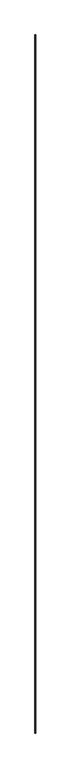
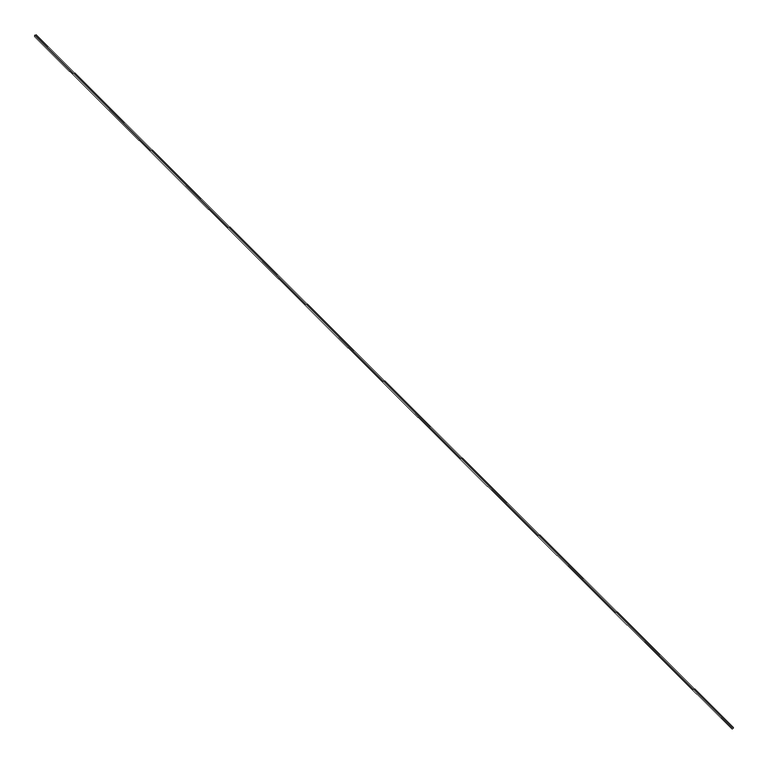
"""IFC4 building model written with IfcOpenShell, lengths in millimetres: proxy geometry, Inner panel:Inner panel:1:Inner panel:1 : Inner panel:Inner panel:300324:2:Inner panel:1:Inner panel:1 : Inner panel:Inner panel:300324:2 : Inner panel:Inner panel:1:Inner panel:1 : Inner panel:Inner panel:300324:300043:57 : Inner panel:Inner panel:1:Inner panel:1 : Inner panel:Inner panel:300324:2:Inner panel:1:Inner panel:1 : Inner panel:Inner panel:300324:2 : Inner panel:Inner panel:1:Inner panel:1 : Inner panel:Inner panel:300324:300043:308120."""

import ifcopenshell
import ifcopenshell.guid

model = None  # the IFC model being written
_history = None  # IfcOwnerHistory: only IFC2X3 demands one
_inside = {}  # id of a spatial element -> (the spatial element, [elements in it])
_under = {}  # id of a project, library or spatial element -> (it, [spatial elements below it])
_declared = {}  # id of a project -> (the project, [libraries it declares])
_typed = {}  # id of a type object -> (the type object, [elements of that type])
_made_of = {}  # id of a material, layer set ... -> (it, [elements and type objects made of it])


def new_model(schema):
    """Start an empty IFC model of exactly this schema.

    Asked for "IFC4X3", IfcOpenShell would pick the latest addendum, in which some entities
    have other attributes; the version numbers below select the first issue.
    IFC2X3 requires an IfcOwnerHistory on every rooted entity: one is made here for all.
    """
    global model, _history
    if schema == "IFC4X3":
        model = ifcopenshell.file(schema_version=(4, 3, 0, 0))
    else:
        model = ifcopenshell.file(schema=schema)
    _inside.clear()
    _under.clear()
    _declared.clear()
    _typed.clear()
    _made_of.clear()
    _history = None
    if model.schema == "IFC2X3":
        org = make("IfcOrganization", Name="unknown")
        user = make(
            "IfcPersonAndOrganization",
            ThePerson=make("IfcPerson", FamilyName="unknown"),
            TheOrganization=org,
        )
        app = make(
            "IfcApplication",
            ApplicationDeveloper=org,
            Version="unknown",
            ApplicationFullName="unknown",
            ApplicationIdentifier="unknown",
        )
        _history = make(
            "IfcOwnerHistory",
            OwningUser=user,
            OwningApplication=app,
            ChangeAction="ADDED",
            CreationDate=0,
        )
    return model


def make(cls, **values):
    """One entity of the class cls with the attributes given. An attribute that is None is left unset."""
    return model.create_entity(
        cls, **{name: value for name, value in values.items() if value is not None}
    )


def rooted(cls, **values):
    """An entity with a GlobalId (a new one), such as an element, a storey or a relation."""
    return make(cls, GlobalId=ifcopenshell.guid.new(), OwnerHistory=_history, **values)


def si_unit(unit_type, name, prefix=None):
    """IfcSIUnit, for example si_unit("LENGTHUNIT", "METRE", prefix="MILLI")."""
    return make("IfcSIUnit", UnitType=unit_type, Prefix=prefix, Name=name)


def assignment(units):
    """IfcUnitAssignment: the units of a project."""
    return None if units is None else make("IfcUnitAssignment", Units=units)


def point(xyz):
    """IfcCartesianPoint."""
    return None if xyz is None else make("IfcCartesianPoint", Coordinates=xyz)


def direction(xyz):
    """IfcDirection."""
    return None if xyz is None else make("IfcDirection", DirectionRatios=xyz)


def frame(location, z_axis=None, x_axis=None):
    """IfcAxis2Placement3D, a coordinate frame: its origin and axes. An axis left out is left unset."""
    return make(
        "IfcAxis2Placement3D",
        Location=point(location),
        Axis=direction(z_axis),
        RefDirection=direction(x_axis),
    )


def origin():
    """The frame at (0, 0, 0) with its axes left unset."""
    return frame((0.0, 0.0, 0.0))


def place(relative_to, where):
    """IfcLocalPlacement: puts the frame where relative to a parent placement (None: the world)."""
    return make(
        "IfcLocalPlacement", PlacementRelTo=relative_to, RelativePlacement=where
    )


def context(
    kind, dimensions, precision=None, world=None, true_north=None, identifier=None
):
    """IfcGeometricRepresentationContext, for example the 3D "Model" context."""
    return make(
        "IfcGeometricRepresentationContext",
        ContextIdentifier=identifier,
        ContextType=kind,
        CoordinateSpaceDimension=dimensions,
        Precision=precision,
        WorldCoordinateSystem=world,
        TrueNorth=true_north,
    )


def project(units=None, contexts=None):
    """IfcProject with its units and contexts."""
    return rooted(
        "IfcProject",
        Name="project",
        RepresentationContexts=contexts,
        UnitsInContext=assignment(units),
    )


def spatial(cls, under=None, at=None, **own):
    """A site, building, storey or space (cls), placed at a placement, below another one or the project."""
    s = rooted(cls, ObjectPlacement=at, **own)
    if under is not None:
        _under.setdefault(under.id(), (under, []))[1].append(s)
    return s


def polyline(points):
    """IfcPolyline through the points."""
    return make("IfcPolyline", Points=[point(p) for p in points])


def outline(outer, holes=None, kind="AREA"):
    """IfcArbitraryClosedProfileDef: a profile drawn as a closed curve; with holes, ...WithVoids."""
    if holes is None:
        return make("IfcArbitraryClosedProfileDef", ProfileType=kind, OuterCurve=outer)
    return make(
        "IfcArbitraryProfileDefWithVoids",
        ProfileType=kind,
        OuterCurve=outer,
        InnerCurves=holes,
    )


def extrude(swept, where, along, depth):
    """IfcExtrudedAreaSolid: the profile swept, set in the frame where, extruded along a direction by depth."""
    return make(
        "IfcExtrudedAreaSolid",
        SweptArea=swept,
        Position=where,
        ExtrudedDirection=direction(along),
        Depth=depth,
    )


def shape(context_of_items, identifier, shape_type, items):
    """IfcShapeRepresentation: the items that make up one representation, for example the "Body"."""
    return make(
        "IfcShapeRepresentation",
        ContextOfItems=context_of_items,
        RepresentationIdentifier=identifier,
        RepresentationType=shape_type,
        Items=items,
    )


def source(mapping_origin, context_of_items, identifier, shape_type, items):
    """IfcRepresentationMap: a shape defined once, which mapped items show again and again."""
    return make(
        "IfcRepresentationMap",
        MappingOrigin=mapping_origin,
        MappedRepresentation=shape(context_of_items, identifier, shape_type, items),
    )


def transform(
    local_origin,
    x_axis=None,
    y_axis=None,
    z_axis=None,
    scale=None,
    scale2=None,
    scale3=None,
    uniform=True,
):
    """IfcCartesianTransformationOperator3D, or its non-uniform kind. x_axis, y_axis, z_axis: its Axis1, 2, 3."""
    if uniform:
        return make(
            "IfcCartesianTransformationOperator3D",
            Axis1=direction(x_axis),
            Axis2=direction(y_axis),
            LocalOrigin=point(local_origin),
            Scale=scale,
            Axis3=direction(z_axis),
        )
    return make(
        "IfcCartesianTransformationOperator3DnonUniform",
        Axis1=direction(x_axis),
        Axis2=direction(y_axis),
        LocalOrigin=point(local_origin),
        Scale=scale,
        Axis3=direction(z_axis),
        Scale2=scale2,
        Scale3=scale3,
    )


def mapped(mapping_source, mapping_target):
    """IfcMappedItem: shows the shape of a source again, moved by a transform."""
    return make(
        "IfcMappedItem", MappingSource=mapping_source, MappingTarget=mapping_target
    )


def made_of(thing, what):
    """Note that an element or type object is made of a material, layer set ...; save() writes the relation."""
    if what is not None:
        _made_of.setdefault(what.id(), (what, []))[1].append(thing)
    return thing


def element(
    cls,
    number,
    at=None,
    inside=None,
    cuts=None,
    type_object=None,
    material=None,
    context=None,
    identifier="Body",
    shape_type=None,
    held_by="IfcProductDefinitionShape",
    body=None,
    shapes=None,
    **own,
):
    """One element of the class cls, such as IfcWall. Its Tag is "e" and its number.

    at: its placement. inside: the storey or other place that contains it. cuts: it is an
    opening in that element (IfcRelVoidsElement). A single representation is given by context,
    identifier, shape_type and body (its items); several are given by shapes. held_by: the class
    of the entity that holds the representations. save() writes the other relations.
    """
    e = rooted(cls, Tag="e%d" % number, ObjectPlacement=at, **own)
    if body is not None:
        shapes = [shape(context, identifier, shape_type, body)]
    if shapes is not None:
        e.Representation = make(held_by, Representations=shapes)
    if inside is not None:
        _inside.setdefault(inside.id(), (inside, []))[1].append(e)
    if cuts is not None:
        rooted(
            "IfcRelVoidsElement", RelatingBuildingElement=cuts, RelatedOpeningElement=e
        )
    if type_object is not None:
        _typed.setdefault(type_object.id(), (type_object, []))[1].append(e)
    return made_of(e, material)


def aggregate(whole, parts):
    """IfcRelAggregates: a whole, such as a stair, and the parts it consists of."""
    return rooted("IfcRelAggregates", RelatingObject=whole, RelatedObjects=parts)


def save(model, path):
    """Write the relations noted so far, then the file.

    IfcRelAggregates (storeys below a building ...), IfcRelContainedInSpatialStructure (elements
    in a storey), IfcRelDefinesByType, IfcRelAssociatesMaterial and IfcRelDeclares: one each for
    every whole, place, type object, material and project.
    """
    for whole, parts in _under.values():
        aggregate(whole, parts)
    for where, things in _inside.values():
        rooted(
            "IfcRelContainedInSpatialStructure",
            RelatedElements=things,
            RelatingStructure=where,
        )
    for kind, things in _typed.values():
        rooted("IfcRelDefinesByType", RelatedObjects=things, RelatingType=kind)
    for what, things in _made_of.values():
        rooted("IfcRelAssociatesMaterial", RelatedObjects=things, RelatingMaterial=what)
    for by, libraries in _declared.values():
        rooted("IfcRelDeclares", RelatingContext=by, RelatedDefinitions=libraries)
    model.write(path)


def generic_models_a7e20831(model_context):
    return source(origin(), model_context, "Body", "SweptSolid", [
        extrude(outline(polyline([(3946.0946172, 560274.3721014), (3943.7154315, 560274.4712342), (3944.3763164, 560290.3324717), (3911.0677176, 560291.72033), (3909.6798593, 560258.4117312), (3942.9884581, 560257.0238729), (3943.649343, 560272.8851104), (3946.0285287, 560272.7859777), (3945.268511, 560254.5455545), (3907.201541, 560256.1316783), (3908.7876647, 560294.1986484), (3946.8546348, 560292.6125246), (3946.0946172, 560274.3721014)])), frame((0.0, -579337.5059673, 0.0), z_axis=(0.0, 1.0, 0.0), x_axis=(0.0, 0.0, 1.0)), (0.0, 0.0, 1.0), 36769.9395833),
    ])


if __name__ == "__main__":
    model = new_model("IFC4")
    model_context = context("Model", 3, world=origin())
    ifc_project = project(units=[si_unit("LENGTHUNIT", "METRE", prefix="MILLI")], contexts=[model_context])
    site = spatial("IfcSite", under=ifc_project)
    building = spatial("IfcBuilding", under=site)
    placement = place(None, origin())
    generic_models_shape = generic_models_a7e20831(model_context)
    element("IfcBuildingElementProxy", 1, Name="Inner panel:Inner panel:1:Inner panel:1 : Inner panel:Inner panel:300324:2:Inner panel:1:Inner panel:1 : Inner panel:Inner panel:300324:2 : Inner panel:Inner panel:1:Inner panel:1 : Inner panel:Inner panel:300324:300043:57 : Inner panel:Inner panel:1:Inner panel:1 : Inner panel:Inner panel:300324:2:Inner panel:1:Inner panel:1 : Inner panel:Inner panel:300324:2 : Inner panel:Inner panel:1:Inner panel:1 : Inner panel:Inner panel:300324:300043:308120", ObjectType="Inner panel:Inner panel:1:Inner panel:1 : Inner panel:Inner panel:300324:2:Inner panel:1:Inner panel:1 : Inner panel:Inner panel:300324:2 : Inner panel:Inner panel:1:Inner panel:1 : Inner panel:Inner panel:300324:300043:57 : Inner panel:Inner panel:1:Inner panel:1 : Inner panel:Inner panel:300324:2:Inner panel:1:Inner panel:1 : Inner panel:Inner panel:300324:2 : Inner panel:Inner panel:1:Inner panel:1 : Inner panel:Inner panel:300324:300043:308120", at=placement, inside=building, context=model_context, shape_type="MappedRepresentation", body=[
        mapped(generic_models_shape, transform((0.0, 0.0, 0.0), x_axis=(1.0, 0.0, 0.0), y_axis=(0.0, 1.0, 0.0), z_axis=(0.0, 0.0, 1.0))),
    ])
    save(model, "model.ifc")

# Revit data of these elements
# Type "Inner panel:Inner panel:1:Inner panel:1 : Inner panel:Inner panel:300324:2:Inner panel:1:Inner panel:1 : Inner panel:Inner panel:300324:2 : Inner panel:Inner panel:1:Inner panel:1 : Inner panel:Inner panel:300324:300043:57 : Inner panel:Inner panel:1:Inner panel:1 : Inner panel:Inner panel:300324:2:Inner panel:1:Inner panel:1 : Inner panel:Inner panel:300324:2 : Inner panel:Inner panel:1:Inner panel:1 : Inner panel:Inner panel:300324:300043:308120"
#   NameOverride = "Inner panel:Inner panel:1:Inner panel:1 : Inner panel:Inner panel:300324:2:Inner panel:1:Inner panel:1 : Inner panel:Inner panel:300324:2 : Inner panel:Inner panel:1:Inner panel:1 : Inner panel:Inner panel:300324:300043:308120"
#   ObjectTypeOverride = "Inner panel:1:Inner panel:1 : Inner panel:Inner panel:300324:2 : Inner panel:Inner panel:1:Inner panel:1 : Inner panel:Inner panel:300324:300043"
#   Reference = "Inner panel"
#   Tag = "308120"
# Element 1 (IfcBuildingElementProxy, "Inner panel:Inner panel:1:Inner panel:1 : Inner panel:Inner panel:300324:2:Inner panel:1:Inner panel:1 : Inner panel:Inner panel:300324:2 : Inner panel:Inner panel:1:Inner panel:1 : Inner panel:Inner panel:300324:300043:57 : Inner panel:Inner panel:1:Inner panel:1 : Inner panel:Inner panel:300324:2:Inner panel:1:Inner panel:1 : Inner panel:Inner panel:300324:2 : Inner panel:Inner panel:1:Inner panel:1 : Inner panel:Inner panel:300324:300043:308120")
#   Materials on its faces: "1 1/2\" X 1 1/2\" SPLIT-SEAM SQUARE TUBING (~24\" CANTILEVER FROM C.L. OF GLULAM)"
# Materials
#   "1 1/2\" X 1 1/2\" SPLIT-SEAM SQUARE TUBING (~24\" CANTILEVER FROM C.L. OF GLULAM)": class "Unassigned", colour RGB 202 201 200, transparency 0, Cost = 0
